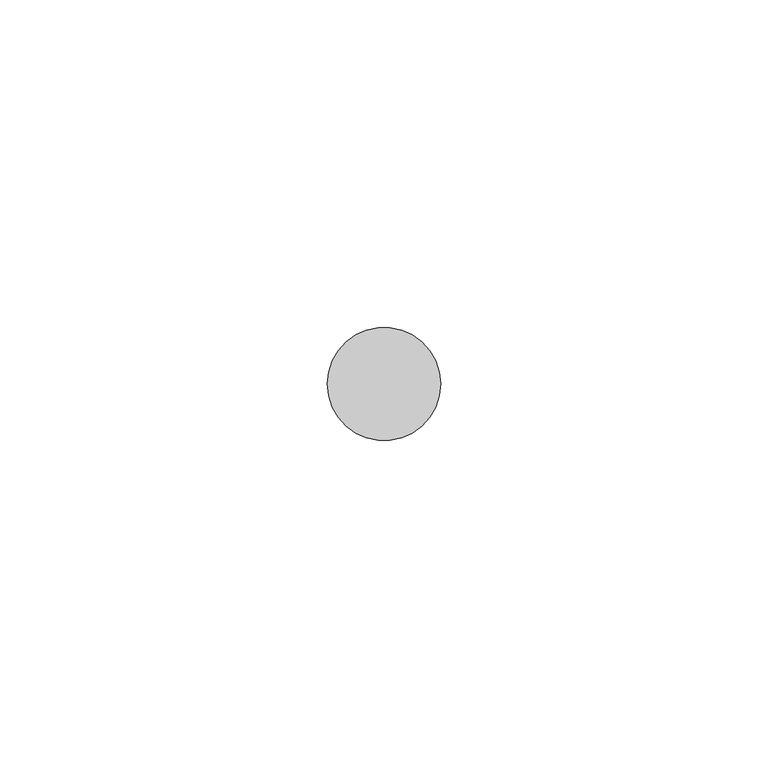
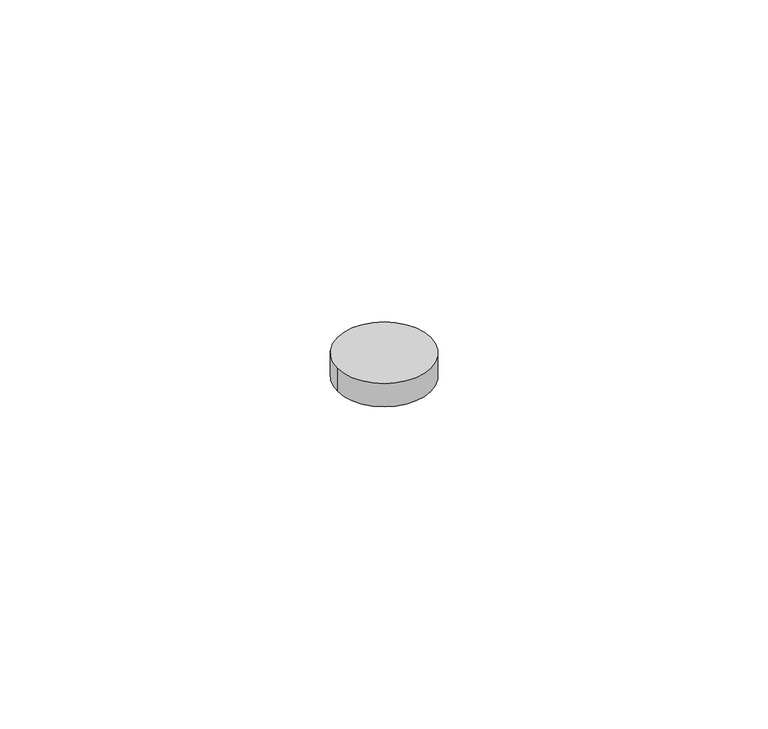
"""IFC4 building model written with IfcOpenShell, lengths in millimetres: proxy geometry, Hinge Pin Keeper8 : Hinge Pin Keeper."""

from ifc_helpers import new_model, si_unit, point, frame, frame_2d, origin, place, context, project, spatial, circle_curve, trimmed, segment, composite_curve, outline, extrude, source, transform, mapped, element, save


def generic_models_657a5c97(model_context):
    return source(origin(), model_context, "Body", "SweptSolid", [
        extrude(outline(composite_curve([segment(trimmed(circle_curve(frame_2d((587319.1320739, -534100.7049841)), 8.6534625), [point((587310.4786114, -534100.7049841))], [point((587327.7855364, -534100.7049841))], False, "CARTESIAN"), True, "CONTINUOUS"), segment(trimmed(circle_curve(frame_2d((587319.1320739, -534100.7049841)), 8.6534625), [point((587327.7855364, -534100.7049841))], [point((587310.4786114, -534100.7049841))], False, "CARTESIAN"), True, "CONTINUOUS")], self_intersect=False)), frame((0.0, 0.0, 1271.7859375), z_axis=(0.0, 0.0, 1.0), x_axis=(1.0, 0.0, 0.0)), (0.0, 0.0, 1.0), 4.5640625),
    ])


if __name__ == "__main__":
    model = new_model("IFC4")
    model_context = context("Model", 3, world=origin())
    ifc_project = project(units=[si_unit("LENGTHUNIT", "METRE", prefix="MILLI")], contexts=[model_context])
    site = spatial("IfcSite", under=ifc_project)
    building = spatial("IfcBuilding", under=site)
    placement = place(None, origin())
    generic_models_shape = generic_models_657a5c97(model_context)
    element("IfcBuildingElementProxy", 1, Name="Hinge Pin Keeper8 : Hinge Pin Keeper", ObjectType="Hinge Pin Keeper8 : Hinge Pin Keeper", at=placement, inside=building, context=model_context, shape_type="MappedRepresentation", body=[
        mapped(generic_models_shape, transform((0.0, 0.0, 0.0), x_axis=(1.0, 0.0, 0.0), y_axis=(0.0, 1.0, 0.0), z_axis=(0.0, 0.0, 1.0))),
    ])
    save(model, "model.ifc")

# Revit data of these elements
# Element 1 (IfcBuildingElementProxy, "Hinge Pin Keeper8 : Hinge Pin Keeper")
#   Materials on its faces: "6\"X6\" WELD-ON STL BUTT HINGE"
# Materials
#   "6\"X6\" WELD-ON STL BUTT HINGE": class "Metal", colour RGB 189 187 185, transparency 0, Description = "Carbon steel", Cost = 0
